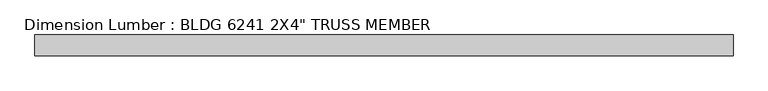
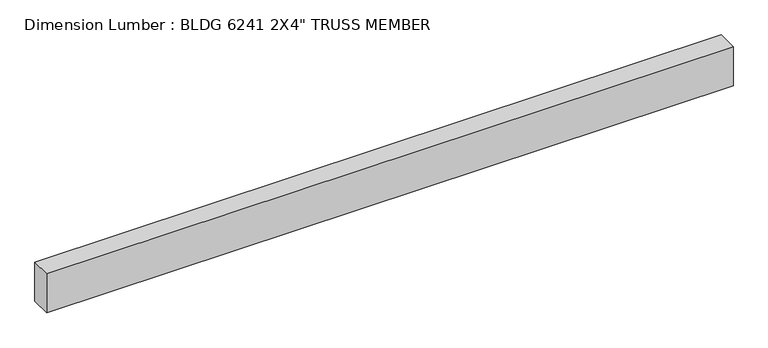
"""IFC4 building model written with IfcOpenShell, lengths in millimetres: beam geometry."""

from ifc_helpers import new_model, si_unit, frame, origin, place, context, project, spatial, polyline, outline, extrude, source, transform, mapped, element, save


def beam_3a1eac92(model_context):
    return source(origin(), model_context, "Body", "SweptSolid", [
        extrude(outline(polyline([(233.4866591, 25.4), (233.4866591, -25.4), (-1464.867127, -25.4), (-1464.867127, 25.4), (233.4866591, 25.4)])), frame((0.0, 0.0, -50.8), z_axis=(0.0, 0.0, 1.0), x_axis=(1.0, 0.0, 0.0)), (0.0, 0.0, 1.0), 101.6),
    ])


if __name__ == "__main__":
    model = new_model("IFC4")
    model_context = context("Model", 3, world=origin())
    ifc_project = project(units=[si_unit("LENGTHUNIT", "METRE", prefix="MILLI")], contexts=[model_context])
    site = spatial("IfcSite", under=ifc_project)
    building = spatial("IfcBuilding", under=site)
    placement = place(None, origin())
    beam_shape = beam_3a1eac92(model_context)
    element("IfcBeam", 1, ObjectType="Dimension Lumber : BLDG 6241 2X4\" TRUSS MEMBER", at=placement, inside=building, context=model_context, shape_type="MappedRepresentation", body=[
        mapped(beam_shape, transform((0.0, 0.0, 0.0), x_axis=(1.0, 0.0, 0.0), y_axis=(0.0, 1.0, 0.0), z_axis=(0.0, 0.0, 1.0))),
    ])
    save(model, "model.ifc")

# Revit data of these elements
# Type "Dimension Lumber : BLDG 6241 2X4\" TRUSS MEMBER"
#   Assembly Code = "B10"
#   A = 0.273472 SF
#   Length [instance default] = 5' - 0"
#   b = 0' - 2"
#   d = 0' - 4"
#   Structural Material [instance default] = Softwood, Lumber
# Element 1 (IfcBeam, "Dimension Lumber : BLDG 6241 2X4\" TRUSS MEMBER")
#   Materials on its faces: "Softwood, Lumber"
# Materials
#   "Softwood, Lumber": class "Wood", colour RGB 223 192 134, transparency 0, Description = "Pinus Echinata", Cost = 0
